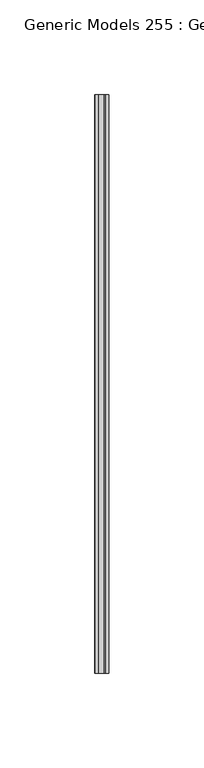
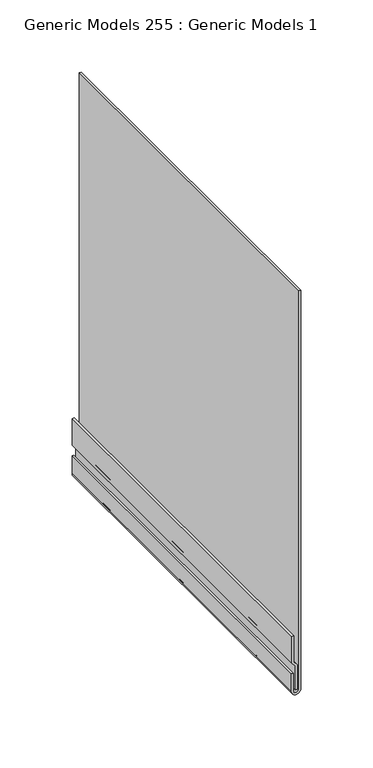
"""IFC4 building model written with IfcOpenShell, lengths in millimetres: proxy geometry, Generic Models 255 : Generic Models 1."""

from ifc_helpers import new_model, si_unit, point, frame, frame_2d, origin, place, context, project, spatial, polyline, circle_curve, trimmed, segment, composite_curve, outline, extrude, source, transform, mapped, element, save


def generic_models_255_generic_models_1_47c10216(model_context):
    return source(origin(), model_context, "Body", "SweptSolid", [
        extrude(outline(composite_curve([segment(trimmed(circle_curve(frame_2d((129335.9319325, 2124.147652)), 3.6737572), [point((129335.9319325, 2120.4738948))], [point((129335.9319325, 2127.8214092))], False, "CARTESIAN"), True, "CONTINUOUS"), segment(polyline([(129335.9319325, 2127.8214092), (129673.8756366, 2127.8214092), (129673.8756366, 2126.2339092), (129335.9319325, 2126.2339092)]), True, "CONTINUOUS"), segment(trimmed(circle_curve(frame_2d((129335.9319325, 2124.147652)), 2.0862572), [point((129335.9319325, 2126.2339092))], [point((129335.9319325, 2122.0613948))], True, "CARTESIAN"), True, "CONTINUOUS"), segment(polyline([(129335.9319325, 2122.0613948), (129351.1841548, 2122.0613948), (129351.1841548, 2120.4738948), (129335.9319325, 2120.4738948)]), True, "CONTINUOUS")], self_intersect=False)), frame((0.0, 5122.2622548, 0.0), z_axis=(0.0, 1.0, 0.0), x_axis=(0.0, 0.0, 1.0)), (0.0, 0.0, 1.0), 304.8),
        extrude(outline(polyline([(129357.2350463, 2125.0676269), (129360.6943174, 2122.3138704), (129382.5923279, 2122.3138704), (129382.5923279, 2120.7263704), (129360.1396021, 2120.7263704), (129356.680331, 2123.4801269), (129336.4315217, 2123.4801269), (129336.4315217, 2125.0676269), (129357.2350463, 2125.0676269)])), frame((0.0, 5122.2622548, 0.0), z_axis=(0.0, 1.0, 0.0), x_axis=(0.0, 0.0, 1.0)), (0.0, 0.0, 1.0), 304.8),
    ])


if __name__ == "__main__":
    model = new_model("IFC4")
    model_context = context("Model", 3, world=origin())
    ifc_project = project(units=[si_unit("LENGTHUNIT", "METRE", prefix="MILLI")], contexts=[model_context])
    site = spatial("IfcSite", under=ifc_project)
    building = spatial("IfcBuilding", under=site)
    placement = place(None, origin())
    generic_models_255_generic_models_1_shape = generic_models_255_generic_models_1_47c10216(model_context)
    element("IfcBuildingElementProxy", 1, Name="Generic Models 255 : Generic Models 1", ObjectType="Generic Models 255 : Generic Models 1", at=placement, inside=building, context=model_context, shape_type="MappedRepresentation", body=[
        mapped(generic_models_255_generic_models_1_shape, transform((0.0, 0.0, 0.0), x_axis=(1.0, 0.0, 0.0), y_axis=(0.0, 1.0, 0.0), z_axis=(0.0, 0.0, 1.0))),
    ])
    save(model, "model.ifc")

# Revit data of these elements
# Element 1 (IfcBuildingElementProxy, "Generic Models 255 : Generic Models 1")
#   Materials on its faces: "_16 GA. COPPER BRAKE METAL FASCIA"
# Materials
#   "_16 GA. COPPER BRAKE METAL FASCIA": class "Generic", colour RGB 175 175 175, transparency 0, Cost = 0
